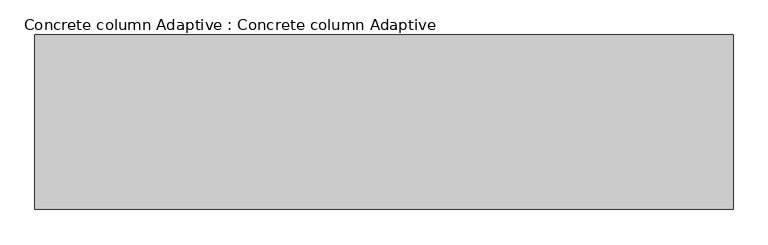
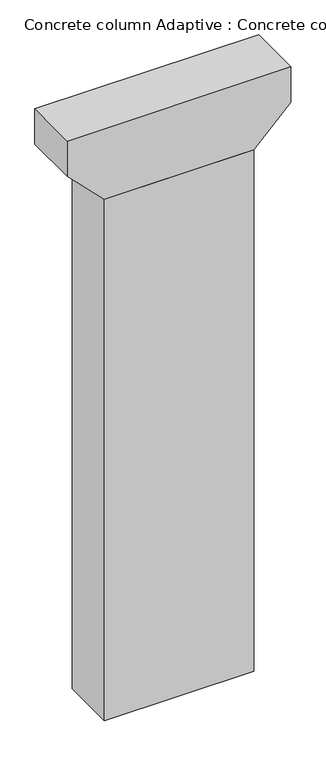
"""IFC4 building model written with IfcOpenShell, lengths in millimetres: proxy geometry, Concrete column Adaptive : Concrete column Adaptive."""

import ifcopenshell
import ifcopenshell.guid

model = None  # the IFC model being written
_history = None  # IfcOwnerHistory: only IFC2X3 demands one
_inside = {}  # id of a spatial element -> (the spatial element, [elements in it])
_under = {}  # id of a project, library or spatial element -> (it, [spatial elements below it])
_declared = {}  # id of a project -> (the project, [libraries it declares])
_typed = {}  # id of a type object -> (the type object, [elements of that type])
_made_of = {}  # id of a material, layer set ... -> (it, [elements and type objects made of it])


def new_model(schema):
    """Start an empty IFC model of exactly this schema.

    Asked for "IFC4X3", IfcOpenShell would pick the latest addendum, in which some entities
    have other attributes; the version numbers below select the first issue.
    IFC2X3 requires an IfcOwnerHistory on every rooted entity: one is made here for all.
    """
    global model, _history
    if schema == "IFC4X3":
        model = ifcopenshell.file(schema_version=(4, 3, 0, 0))
    else:
        model = ifcopenshell.file(schema=schema)
    _inside.clear()
    _under.clear()
    _declared.clear()
    _typed.clear()
    _made_of.clear()
    _history = None
    if model.schema == "IFC2X3":
        org = make("IfcOrganization", Name="unknown")
        user = make(
            "IfcPersonAndOrganization",
            ThePerson=make("IfcPerson", FamilyName="unknown"),
            TheOrganization=org,
        )
        app = make(
            "IfcApplication",
            ApplicationDeveloper=org,
            Version="unknown",
            ApplicationFullName="unknown",
            ApplicationIdentifier="unknown",
        )
        _history = make(
            "IfcOwnerHistory",
            OwningUser=user,
            OwningApplication=app,
            ChangeAction="ADDED",
            CreationDate=0,
        )
    return model


def make(cls, **values):
    """One entity of the class cls with the attributes given. An attribute that is None is left unset."""
    return model.create_entity(
        cls, **{name: value for name, value in values.items() if value is not None}
    )


def rooted(cls, **values):
    """An entity with a GlobalId (a new one), such as an element, a storey or a relation."""
    return make(cls, GlobalId=ifcopenshell.guid.new(), OwnerHistory=_history, **values)


def si_unit(unit_type, name, prefix=None):
    """IfcSIUnit, for example si_unit("LENGTHUNIT", "METRE", prefix="MILLI")."""
    return make("IfcSIUnit", UnitType=unit_type, Prefix=prefix, Name=name)


def assignment(units):
    """IfcUnitAssignment: the units of a project."""
    return None if units is None else make("IfcUnitAssignment", Units=units)


def point(xyz):
    """IfcCartesianPoint."""
    return None if xyz is None else make("IfcCartesianPoint", Coordinates=xyz)


def direction(xyz):
    """IfcDirection."""
    return None if xyz is None else make("IfcDirection", DirectionRatios=xyz)


def frame(location, z_axis=None, x_axis=None):
    """IfcAxis2Placement3D, a coordinate frame: its origin and axes. An axis left out is left unset."""
    return make(
        "IfcAxis2Placement3D",
        Location=point(location),
        Axis=direction(z_axis),
        RefDirection=direction(x_axis),
    )


def origin():
    """The frame at (0, 0, 0) with its axes left unset."""
    return frame((0.0, 0.0, 0.0))


def origin_with_axes():
    """The frame at (0, 0, 0) with the z axis (0, 0, 1) and the x axis (1, 0, 0) written out."""
    return frame((0.0, 0.0, 0.0), z_axis=(0.0, 0.0, 1.0), x_axis=(1.0, 0.0, 0.0))


def place(relative_to, where):
    """IfcLocalPlacement: puts the frame where relative to a parent placement (None: the world)."""
    return make(
        "IfcLocalPlacement", PlacementRelTo=relative_to, RelativePlacement=where
    )


def context(
    kind, dimensions, precision=None, world=None, true_north=None, identifier=None
):
    """IfcGeometricRepresentationContext, for example the 3D "Model" context."""
    return make(
        "IfcGeometricRepresentationContext",
        ContextIdentifier=identifier,
        ContextType=kind,
        CoordinateSpaceDimension=dimensions,
        Precision=precision,
        WorldCoordinateSystem=world,
        TrueNorth=true_north,
    )


def project(units=None, contexts=None):
    """IfcProject with its units and contexts."""
    return rooted(
        "IfcProject",
        Name="project",
        RepresentationContexts=contexts,
        UnitsInContext=assignment(units),
    )


def spatial(cls, under=None, at=None, **own):
    """A site, building, storey or space (cls), placed at a placement, below another one or the project."""
    s = rooted(cls, ObjectPlacement=at, **own)
    if under is not None:
        _under.setdefault(under.id(), (under, []))[1].append(s)
    return s


def polyline(points):
    """IfcPolyline through the points."""
    return make("IfcPolyline", Points=[point(p) for p in points])


def outline(outer, holes=None, kind="AREA"):
    """IfcArbitraryClosedProfileDef: a profile drawn as a closed curve; with holes, ...WithVoids."""
    if holes is None:
        return make("IfcArbitraryClosedProfileDef", ProfileType=kind, OuterCurve=outer)
    return make(
        "IfcArbitraryProfileDefWithVoids",
        ProfileType=kind,
        OuterCurve=outer,
        InnerCurves=holes,
    )


def extrude(swept, where, along, depth):
    """IfcExtrudedAreaSolid: the profile swept, set in the frame where, extruded along a direction by depth."""
    return make(
        "IfcExtrudedAreaSolid",
        SweptArea=swept,
        Position=where,
        ExtrudedDirection=direction(along),
        Depth=depth,
    )


def shape(context_of_items, identifier, shape_type, items):
    """IfcShapeRepresentation: the items that make up one representation, for example the "Body"."""
    return make(
        "IfcShapeRepresentation",
        ContextOfItems=context_of_items,
        RepresentationIdentifier=identifier,
        RepresentationType=shape_type,
        Items=items,
    )


def source(mapping_origin, context_of_items, identifier, shape_type, items):
    """IfcRepresentationMap: a shape defined once, which mapped items show again and again."""
    return make(
        "IfcRepresentationMap",
        MappingOrigin=mapping_origin,
        MappedRepresentation=shape(context_of_items, identifier, shape_type, items),
    )


def transform(
    local_origin,
    x_axis=None,
    y_axis=None,
    z_axis=None,
    scale=None,
    scale2=None,
    scale3=None,
    uniform=True,
):
    """IfcCartesianTransformationOperator3D, or its non-uniform kind. x_axis, y_axis, z_axis: its Axis1, 2, 3."""
    if uniform:
        return make(
            "IfcCartesianTransformationOperator3D",
            Axis1=direction(x_axis),
            Axis2=direction(y_axis),
            LocalOrigin=point(local_origin),
            Scale=scale,
            Axis3=direction(z_axis),
        )
    return make(
        "IfcCartesianTransformationOperator3DnonUniform",
        Axis1=direction(x_axis),
        Axis2=direction(y_axis),
        LocalOrigin=point(local_origin),
        Scale=scale,
        Axis3=direction(z_axis),
        Scale2=scale2,
        Scale3=scale3,
    )


def mapped(mapping_source, mapping_target):
    """IfcMappedItem: shows the shape of a source again, moved by a transform."""
    return make(
        "IfcMappedItem", MappingSource=mapping_source, MappingTarget=mapping_target
    )


def made_of(thing, what):
    """Note that an element or type object is made of a material, layer set ...; save() writes the relation."""
    if what is not None:
        _made_of.setdefault(what.id(), (what, []))[1].append(thing)
    return thing


def element(
    cls,
    number,
    at=None,
    inside=None,
    cuts=None,
    type_object=None,
    material=None,
    context=None,
    identifier="Body",
    shape_type=None,
    held_by="IfcProductDefinitionShape",
    body=None,
    shapes=None,
    **own,
):
    """One element of the class cls, such as IfcWall. Its Tag is "e" and its number.

    at: its placement. inside: the storey or other place that contains it. cuts: it is an
    opening in that element (IfcRelVoidsElement). A single representation is given by context,
    identifier, shape_type and body (its items); several are given by shapes. held_by: the class
    of the entity that holds the representations. save() writes the other relations.
    """
    e = rooted(cls, Tag="e%d" % number, ObjectPlacement=at, **own)
    if body is not None:
        shapes = [shape(context, identifier, shape_type, body)]
    if shapes is not None:
        e.Representation = make(held_by, Representations=shapes)
    if inside is not None:
        _inside.setdefault(inside.id(), (inside, []))[1].append(e)
    if cuts is not None:
        rooted(
            "IfcRelVoidsElement", RelatingBuildingElement=cuts, RelatedOpeningElement=e
        )
    if type_object is not None:
        _typed.setdefault(type_object.id(), (type_object, []))[1].append(e)
    return made_of(e, material)


def aggregate(whole, parts):
    """IfcRelAggregates: a whole, such as a stair, and the parts it consists of."""
    return rooted("IfcRelAggregates", RelatingObject=whole, RelatedObjects=parts)


def save(model, path):
    """Write the relations noted so far, then the file.

    IfcRelAggregates (storeys below a building ...), IfcRelContainedInSpatialStructure (elements
    in a storey), IfcRelDefinesByType, IfcRelAssociatesMaterial and IfcRelDeclares: one each for
    every whole, place, type object, material and project.
    """
    for whole, parts in _under.values():
        aggregate(whole, parts)
    for where, things in _inside.values():
        rooted(
            "IfcRelContainedInSpatialStructure",
            RelatedElements=things,
            RelatingStructure=where,
        )
    for kind, things in _typed.values():
        rooted("IfcRelDefinesByType", RelatedObjects=things, RelatingType=kind)
    for what, things in _made_of.values():
        rooted("IfcRelAssociatesMaterial", RelatedObjects=things, RelatingMaterial=what)
    for by, libraries in _declared.values():
        rooted("IfcRelDeclares", RelatingContext=by, RelatedDefinitions=libraries)
    model.write(path)


def concrete_column_adaptive_concrete_column_adaptive_048184f4(model_context):
    return source(origin(), model_context, "Body", "SweptSolid", [
        extrude(outline(polyline([(33587.0, 6000.0), (33587.0, -6000.0), (31587.0, -6000.0), (29587.0, -4000.0), (29587.0, 4000.0), (31587.0, 6000.0), (33587.0, 6000.0)])), frame((0.0, -1500.0, 0.0), z_axis=(0.0, 1.0, 0.0), x_axis=(0.0, 0.0, 1.0)), (0.0, 0.0, 1.0), 3000.0),
        extrude(outline(polyline([(-4000.0, -1500.0), (-4000.0, 1500.0), (4000.0, 1500.0), (4000.0, -1500.0), (-4000.0, -1500.0)])), origin_with_axes(), (0.0, 0.0, 1.0), 29587.0),
    ])


if __name__ == "__main__":
    model = new_model("IFC4")
    model_context = context("Model", 3, world=origin())
    ifc_project = project(units=[si_unit("LENGTHUNIT", "METRE", prefix="MILLI")], contexts=[model_context])
    site = spatial("IfcSite", under=ifc_project)
    building = spatial("IfcBuilding", under=site)
    placement = place(None, origin())
    concrete_column_adaptive_concrete_column_adaptive_shape = concrete_column_adaptive_concrete_column_adaptive_048184f4(model_context)
    element("IfcBuildingElementProxy", 1, Name="Concrete column Adaptive : Concrete column Adaptive", ObjectType="Concrete column Adaptive : Concrete column Adaptive", at=placement, inside=building, context=model_context, shape_type="MappedRepresentation", body=[
        mapped(concrete_column_adaptive_concrete_column_adaptive_shape, transform((0.0, 0.0, 0.0), x_axis=(1.0, 0.0, 0.0), y_axis=(0.0, 1.0, 0.0), z_axis=(0.0, 0.0, 1.0))),
    ])
    save(model, "model.ifc")

# Revit data of these elements
# Type "Concrete column Adaptive : Concrete column Adaptive"
#   Height [instance default] = 30000 mm
#   Default Elevation = 0
# Element 1 (IfcBuildingElementProxy, "Concrete column Adaptive : Concrete column Adaptive")
#   Height = 29587 mm
